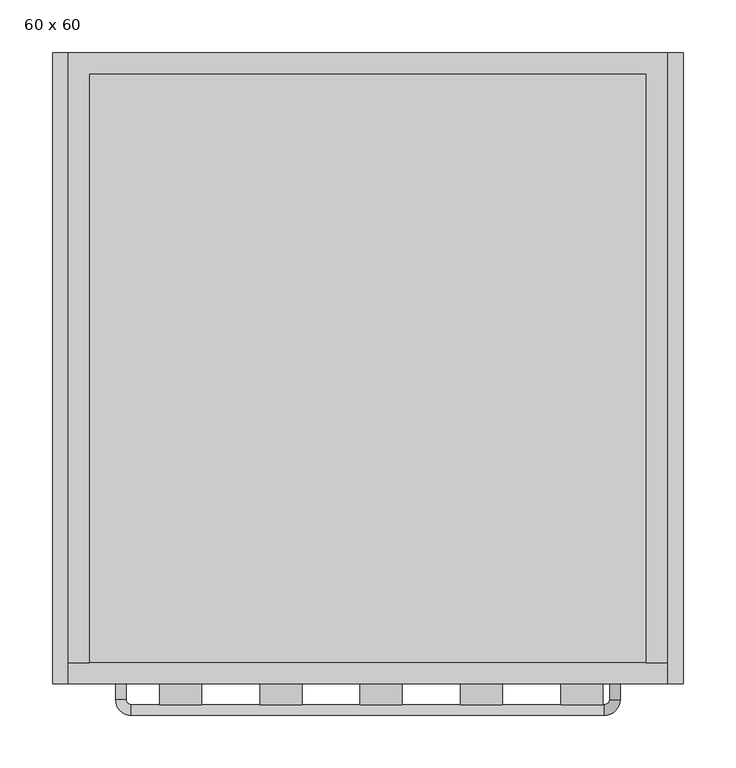
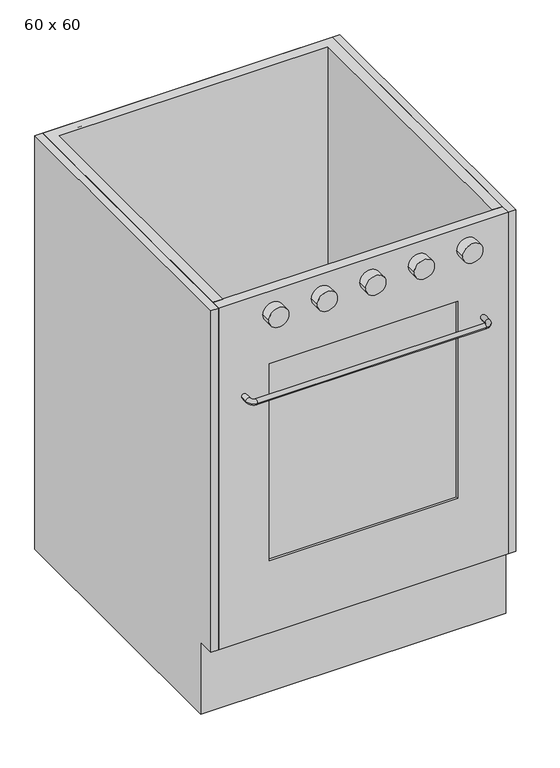
"""IFC4 building model written with IfcOpenShell, lengths in millimetres: furniture geometry, Unterschrank - Mit Einbaubackofen : 60 x 60."""

from ifc_helpers import new_model, si_unit, point, frame, frame_2d, origin, place, context, project, spatial, polyline, circle_curve, ellipse_curve, trimmed, segment, composite_curve, outline, extrude, faceted_brep, source, transform, mapped, element, save
from ifc_brep_helpers import plane_surface, cylinder_surface, revolved_surface, advanced_brep


def furniture_60_x_60_7f890a1d(model_context):
    return source(origin(), model_context, "Body", "SolidModel", [
        advanced_brep(
        [(248.7377049, -600.0, 660.0), (258.7377049, -600.0, 660.0), (248.7377049, -615.094, 660.0), (258.7377049, -615.094, 660.0), (243.8317049, -630.0, 660.0), (243.8317049, -620.0, 660.0), (-206.3562951, -620.0, 660.0), (-206.3562951, -630.0, 660.0), (-221.2622951, -615.094, 660.0), (-211.2622951, -615.094, 660.0), (-211.2622951, -600.0, 660.0), (-221.2622951, -600.0, 660.0)],
        [
            (0, 1, circle_curve(frame((253.7377049, -600.0, 660.0), z_axis=(0.0, 1.0, 0.0), x_axis=(1.0, 0.0, 0.0)), 5.0)),
            (1, 0, circle_curve(frame((253.7377049, -600.0, 660.0), z_axis=(0.0, 1.0, 0.0), x_axis=(1.0, 0.0, 0.0)), 5.0)),
            (0, 2),
            (2, 3, circle_curve(frame((253.7377049, -615.094, 660.0), z_axis=(0.0, 1.0, 0.0), x_axis=(1.0, 0.0, 0.0)), 5.0)),
            (3, 1),
            (3, 2, circle_curve(frame((253.7377049, -615.094, 660.0), z_axis=(0.0, 1.0, 0.0), x_axis=(1.0, 0.0, 0.0)), 5.0)),
            (4, 3, circle_curve(frame((243.8317049, -615.094, 660.0), z_axis=(0.0, 0.0, 1.0), x_axis=(1.0, 0.0, 0.0)), 14.906)),
            (2, 5, circle_curve(frame((243.8317049, -615.094, 660.0), z_axis=(0.0, 0.0, -1.0), x_axis=(1.0, 0.0, 0.0)), 4.906)),
            (5, 4, circle_curve(frame((243.8317049, -625.0, 660.0), z_axis=(1.0, 0.0, 0.0), x_axis=(0.0, -1.0, 0.0)), 5.0)),
            (4, 5, circle_curve(frame((243.8317049, -625.0, 660.0), z_axis=(1.0, 0.0, 0.0), x_axis=(0.0, -1.0, 0.0)), 5.0)),
            (5, 6),
            (6, 7, circle_curve(frame((-206.3562951, -625.0, 660.0), z_axis=(1.0, 0.0, 0.0), x_axis=(0.0, -1.0, 0.0)), 5.0)),
            (7, 4),
            (7, 6, circle_curve(frame((-206.3562951, -625.0, 660.0), z_axis=(1.0, 0.0, 0.0), x_axis=(0.0, -1.0, 0.0)), 5.0)),
            (8, 7, circle_curve(frame((-206.3562951, -615.094, 660.0), z_axis=(0.0, 0.0, 1.0), x_axis=(0.0, -1.0, 0.0)), 14.906)),
            (6, 9, circle_curve(frame((-206.3562951, -615.094, 660.0), z_axis=(0.0, 0.0, -1.0), x_axis=(0.0, -1.0, 0.0)), 4.906)),
            (9, 8, circle_curve(frame((-216.2622951, -615.094, 660.0), z_axis=(0.0, -1.0, 0.0), x_axis=(-1.0, 0.0, 0.0)), 5.0)),
            (8, 9, circle_curve(frame((-216.2622951, -615.094, 660.0), z_axis=(0.0, -1.0, 0.0), x_axis=(-1.0, 0.0, 0.0)), 5.0)),
            (10, 11, circle_curve(frame((-216.2622951, -600.0, 660.0), z_axis=(0.0, 1.0, 0.0), x_axis=(-1.0, 0.0, 0.0)), 5.0)),
            (11, 10, circle_curve(frame((-216.2622951, -600.0, 660.0), z_axis=(0.0, 1.0, 0.0), x_axis=(-1.0, 0.0, 0.0)), 5.0)),
            (9, 10),
            (11, 8),
        ],
        [
            plane_surface(frame((253.7377049, -600.0, 660.0), z_axis=(0.0, 1.0, 0.0), x_axis=(0.0, 0.0, 1.0))),
            cylinder_surface(frame((253.7377049, -600.0, 660.0), z_axis=(0.0, 1.0, 0.0), x_axis=(1.0, 0.0, 0.0)), 5.0),
            revolved_surface(trimmed(ellipse_curve(frame((253.7377049, -615.094, 660.0), z_axis=(0.0, 1.0, 0.0), x_axis=(1.0, 0.0, 0.0)), 5.0, 5.0), [point((248.7377049, -615.094, 660.0))], [point((258.7377049, -615.094, 660.0))], True, "CARTESIAN"), (243.8317049, -615.094, 660.0), (0.0, 0.0, -1.0)),
            revolved_surface(trimmed(ellipse_curve(frame((253.7377049, -615.094, 660.0), z_axis=(0.0, 1.0, 0.0), x_axis=(1.0, 0.0, 0.0)), 5.0, 5.0), [point((258.7377049, -615.094, 660.0))], [point((248.7377049, -615.094, 660.0))], True, "CARTESIAN"), (243.8317049, -615.094, 660.0), (0.0, 0.0, -1.0)),
            cylinder_surface(frame((243.8317049, -625.0, 660.0), z_axis=(1.0, 0.0, 0.0), x_axis=(0.0, -1.0, 0.0)), 5.0),
            revolved_surface(trimmed(ellipse_curve(frame((-206.3562951, -625.0, 660.0), z_axis=(1.0, 0.0, 0.0), x_axis=(0.0, -1.0, 0.0)), 5.0, 5.0), [point((-206.3562951, -620.0, 660.0))], [point((-206.3562951, -630.0, 660.0))], True, "CARTESIAN"), (-206.3562951, -615.094, 660.0), (0.0, 0.0, -1.0)),
            revolved_surface(trimmed(ellipse_curve(frame((-206.3562951, -625.0, 660.0), z_axis=(1.0, 0.0, 0.0), x_axis=(0.0, -1.0, 0.0)), 5.0, 5.0), [point((-206.3562951, -630.0, 660.0))], [point((-206.3562951, -620.0, 660.0))], True, "CARTESIAN"), (-206.3562951, -615.094, 660.0), (0.0, 0.0, -1.0)),
            plane_surface(frame((-216.2622951, -600.0, 660.0), z_axis=(0.0, 1.0, 0.0), x_axis=(0.0, 0.0, 1.0))),
            cylinder_surface(frame((-216.2622951, -615.094, 660.0), z_axis=(0.0, -1.0, 0.0), x_axis=(-1.0, 0.0, 0.0)), 5.0),
        ],
        [
            (0, [[1, 2]]),
            (1, [[-1, 3, 4, 5]]),
            (1, [[-2, -5, 6, -3]]),
            (2, [[7, -4, 8, 9]]),
            (3, [[-8, -6, -7, 10]]),
            (4, [[-9, 11, 12, 13]]),
            (4, [[-10, -13, 14, -11]]),
            (5, [[15, -12, 16, 17]]),
            (6, [[-16, -14, -15, 18]]),
            (7, [[19, 20]]),
            (8, [[-17, 21, -20, 22]]),
            (8, [[-18, -22, -19, -21]]),
        ],
    ),
        faceted_brep([(-246.2622951, -580.0, 180.0), (283.7377049, -580.0, 180.0), (283.7377049, -20.0, 180.0), (-246.2622951, -20.0, 180.0), (-266.2622951, -580.0, 150.0), (-266.2622951, 0.0, 150.0), (303.7377049, 0.0, 150.0), (303.7377049, -580.0, 150.0), (-246.2622951, -580.0, 860.0), (-266.2622951, -580.0, 860.0), (303.7377049, -580.0, 860.0), (283.7377049, -580.0, 860.0), (283.7377049, -20.0, 860.0), (303.7377049, 0.0, 860.0), (-266.2622951, 0.0, 860.0), (-246.2622951, -20.0, 860.0)], [[[0, 1, 2, 3]], [[4, 5, 6, 7]], [[1, 0, 8, 9, 4, 7, 10, 11]], [[12, 11, 10, 13, 14, 9, 8, 15]], [[11, 12, 2, 1]], [[13, 10, 7, 6]], [[14, 13, 6, 5]], [[9, 14, 5, 4]], [[15, 8, 0, 3]], [[12, 15, 3, 2]]]),
        extrude(outline(composite_curve([segment(trimmed(circle_curve(frame_2d((815.8278501, -159.4390198)), 20.0), [point((815.8278501, -179.4390198))], [point((815.8278501, -139.4390198))], False, "CARTESIAN"), True, "CONTINUOUS"), segment(trimmed(circle_curve(frame_2d((815.8278501, -159.4390198)), 20.0), [point((815.8278501, -139.4390198))], [point((815.8278501, -179.4390198))], False, "CARTESIAN"), True, "CONTINUOUS")], self_intersect=False)), frame((0.0, -620.0, 0.0), z_axis=(0.0, 1.0, 0.0), x_axis=(0.0, 0.0, 1.0)), (0.0, 0.0, 1.0), 20.0),
        extrude(outline(composite_curve([segment(trimmed(circle_curve(frame_2d((815.8278501, -64.0223532)), 20.0), [point((815.8278501, -84.0223532))], [point((815.8278501, -44.0223532))], False, "CARTESIAN"), True, "CONTINUOUS"), segment(trimmed(circle_curve(frame_2d((815.8278501, -64.0223532)), 20.0), [point((815.8278501, -44.0223532))], [point((815.8278501, -84.0223532))], False, "CARTESIAN"), True, "CONTINUOUS")], self_intersect=False)), frame((0.0, -620.0, 0.0), z_axis=(0.0, 1.0, 0.0), x_axis=(0.0, 0.0, 1.0)), (0.0, 0.0, 1.0), 20.0),
        extrude(outline(composite_curve([segment(trimmed(circle_curve(frame_2d((815.8278501, 31.3943135)), 20.0), [point((815.8278501, 11.3943135))], [point((815.8278501, 51.3943135))], False, "CARTESIAN"), True, "CONTINUOUS"), segment(trimmed(circle_curve(frame_2d((815.8278501, 31.3943135)), 20.0), [point((815.8278501, 51.3943135))], [point((815.8278501, 11.3943135))], False, "CARTESIAN"), True, "CONTINUOUS")], self_intersect=False)), frame((0.0, -620.0, 0.0), z_axis=(0.0, 1.0, 0.0), x_axis=(0.0, 0.0, 1.0)), (0.0, 0.0, 1.0), 20.0),
        extrude(outline(composite_curve([segment(trimmed(circle_curve(frame_2d((815.8278501, 126.8109802)), 20.0), [point((815.8278501, 106.8109802))], [point((815.8278501, 146.8109802))], False, "CARTESIAN"), True, "CONTINUOUS"), segment(trimmed(circle_curve(frame_2d((815.8278501, 126.8109802)), 20.0), [point((815.8278501, 146.8109802))], [point((815.8278501, 106.8109802))], False, "CARTESIAN"), True, "CONTINUOUS")], self_intersect=False)), frame((0.0, -620.0, 0.0), z_axis=(0.0, 1.0, 0.0), x_axis=(0.0, 0.0, 1.0)), (0.0, 0.0, 1.0), 20.0),
        extrude(outline(composite_curve([segment(trimmed(circle_curve(frame_2d((815.8278501, 222.2276468)), 20.0), [point((815.8278501, 202.2276468))], [point((815.8278501, 242.2276468))], False, "CARTESIAN"), True, "CONTINUOUS"), segment(trimmed(circle_curve(frame_2d((815.8278501, 222.2276468)), 20.0), [point((815.8278501, 242.2276468))], [point((815.8278501, 202.2276468))], False, "CARTESIAN"), True, "CONTINUOUS")], self_intersect=False)), frame((0.0, -620.0, 0.0), z_axis=(0.0, 1.0, 0.0), x_axis=(0.0, 0.0, 1.0)), (0.0, 0.0, 1.0), 20.0),
        extrude(outline(polyline([(203.7377049, -585.0), (203.7377049, -595.0), (-166.2622951, -595.0), (-166.2622951, -585.0), (203.7377049, -585.0)])), frame((0.0, 0.0, 300.0), z_axis=(0.0, 0.0, 1.0), x_axis=(1.0, 0.0, 0.0)), (0.0, 0.0, 1.0), 410.0),
        extrude(outline(polyline([(860.0, -266.2622951), (150.0, -266.2622951), (150.0, 303.7377049), (860.0, 303.7377049), (860.0, -266.2622951)]), holes=[polyline([(710.0, 203.7377049), (300.0, 203.7377049), (300.0, -166.2622951), (710.0, -166.2622951), (710.0, 203.7377049)])]), frame((0.0, -600.0, 0.0), z_axis=(0.0, 1.0, 0.0), x_axis=(0.0, 0.0, 1.0)), (0.0, 0.0, 1.0), 20.0),
        faceted_brep([(-266.2622951, -600.0, 860.0), (-266.2622951, -15.0, 860.0), (303.7377049, -15.0, 860.0), (303.7377049, -600.0, 860.0), (318.7377049, -600.0, 860.0), (318.7377049, 0.0, 860.0), (-281.2622951, 0.0, 860.0), (-281.2622951, -600.0, 860.0), (-266.2622951, -600.0, 150.0), (-281.2622951, -600.0, 150.0), (-281.2622951, -565.0, 150.0), (-266.2622951, -565.0, 150.0), (318.7377049, -600.0, 150.0), (303.7377049, -600.0, 150.0), (303.7377049, -565.0, 150.0), (318.7377049, -565.0, 150.0), (-266.2622951, -15.0, 150.0), (303.7377049, -15.0, 150.0), (318.7377049, -565.0, 0.0), (318.7377049, 0.0, 0.0), (-281.2622951, 0.0, 0.0), (-281.2622951, -565.0, 0.0)], [[[0, 1, 2, 3, 4, 5, 6, 7]], [[8, 9, 10, 11]], [[12, 13, 14, 15]], [[1, 0, 8, 11, 16]], [[2, 1, 16, 17]], [[3, 2, 17, 14, 13]], [[5, 4, 12, 15, 18, 19]], [[6, 5, 19, 20]], [[7, 6, 20, 21, 10, 9]], [[0, 7, 9, 8]], [[11, 14, 17, 16]], [[19, 18, 21, 20]], [[21, 18, 15, 14, 11, 10]], [[4, 3, 13, 12]]]),
    ])


if __name__ == "__main__":
    model = new_model("IFC4")
    model_context = context("Model", 3, world=origin())
    ifc_project = project(units=[si_unit("LENGTHUNIT", "METRE", prefix="MILLI")], contexts=[model_context])
    site = spatial("IfcSite", under=ifc_project)
    building = spatial("IfcBuilding", under=site)
    placement = place(None, origin())
    furniture_60_x_60_shape = furniture_60_x_60_7f890a1d(model_context)
    element("IfcFurniture", 1, ObjectType="Unterschrank - Mit Einbaubackofen : 60 x 60", at=placement, inside=building, context=model_context, shape_type="MappedRepresentation", body=[
        mapped(furniture_60_x_60_shape, transform((0.0, 0.0, 0.0), x_axis=(1.0, 0.0, 0.0), y_axis=(0.0, 1.0, 0.0), z_axis=(0.0, 0.0, 1.0))),
    ])
    save(model, "model.ifc")

# Revit data of these elements
# Type "Unterschrank - Mit Einbaubackofen : 60 x 60"
#   Depth = 0.600 m
#   Height = 0.860 m
#   Sockeltiefe = 0.035 m
#   Sockelhöhe = 0.150 m
#   Width = 0.600 m
#   Höhe Backofen = 0.860 m
#   Breite Backofen = 0.570 m
#   Corpus = Kunststoff - Glatt - Weiß
#   Griff = Metall - Aluminium
#   Backofen = Metall - Aluminium
# Element 1 (IfcFurniture, "Unterschrank - Mit Einbaubackofen : 60 x 60")
#   Materials on its faces: "Metall - Aluminium", "Kunststoff - Glatt - Weiß", "Glas"
# Materials
#   "Kunststoff - Glatt - Weiß": class "Metall", colour RGB 234 234 234, transparency 0
#   "Metall - Aluminium": class "Metall", colour RGB 247 247 247, transparency 0, Description = "Aluminium 6061", Cost = 0
#   "Glas": class "Glas", colour RGB 0 0 255, transparency 0.75, Comments = "Render-Darstellung nicht aktualisiert ", Cost = 0
